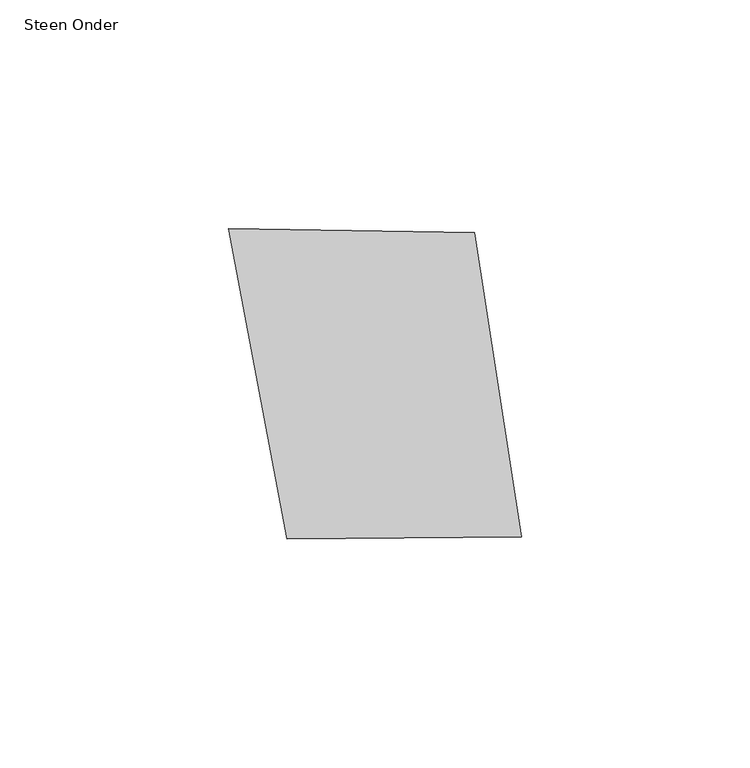
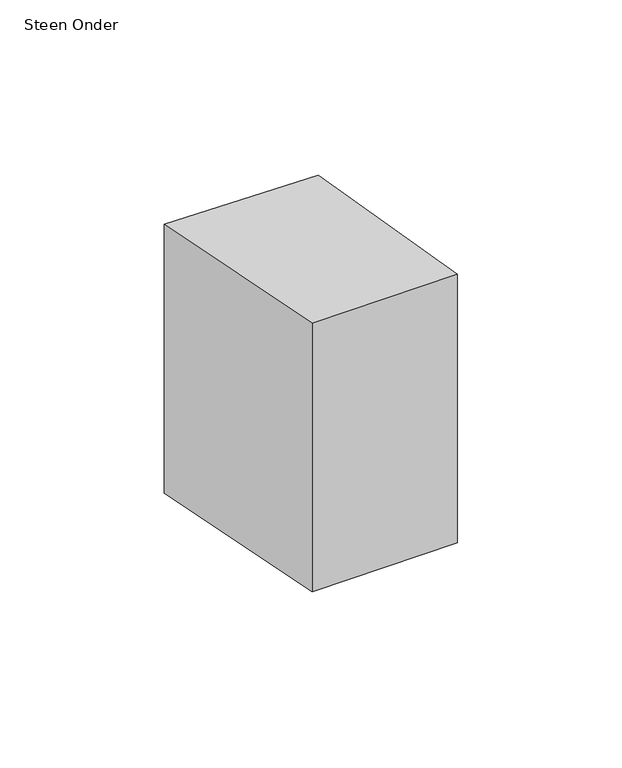
"""IFC4 building model written with IfcOpenShell, lengths in millimetres: proxy geometry, 00_GMA_steen_versie_4 : Steen Onder."""

from ifc_helpers import new_model, si_unit, origin, origin_with_axes, place, context, project, spatial, polyline, outline, extrude, source, transform, mapped, element, save


def steen_onder_d345ffee(model_context):
    return source(origin(), model_context, "Body", "SweptSolid", [
        extrude(outline(polyline([(95.7779209, 99.5138941), (106.0949539, 32.874146), (54.8034129, 32.4112295), (41.9456954, 100.3821665), (95.7779209, 99.5138941)])), origin_with_axes(), (0.0, 0.0, 1.0), 100.0),
    ])


if __name__ == "__main__":
    model = new_model("IFC4")
    model_context = context("Model", 3, world=origin())
    ifc_project = project(units=[si_unit("LENGTHUNIT", "METRE", prefix="MILLI")], contexts=[model_context])
    site = spatial("IfcSite", under=ifc_project)
    building = spatial("IfcBuilding", under=site)
    placement = place(None, origin())
    steen_onder_shape = steen_onder_d345ffee(model_context)
    element("IfcBuildingElementProxy", 1, Name="00_GMA_steen_versie_4 : Steen Onder", ObjectType="00_GMA_steen_versie_4 : Steen Onder", at=placement, inside=building, context=model_context, shape_type="MappedRepresentation", body=[
        mapped(steen_onder_shape, transform((0.0, 0.0, 0.0), x_axis=(1.0, 0.0, 0.0), y_axis=(0.0, 1.0, 0.0), z_axis=(0.0, 0.0, 1.0))),
    ])
    save(model, "model.ifc")

# Revit data of these elements
# Type "00_GMA_steen_versie_4 : Steen Onder"
#   StootVoegHalfBoven [instance default] = 5 mm
#   StootVoegHalf [instance default] = 5 mm
#   StootVoegBreedteOnder = 10 mm
#   StootVoegBreedteBoven = 10 mm
#   Steendikte = 100 mm
#   LintVoegOnderHalf = 0 mm
#   LintVoegOnder = 0 mm
#   LintVoegBovenHalf = 5 mm
#   LintVoegBoven = 10 mm
#   materiaal = none
#   MateriaalVoeg = none
#   Default Elevation = 0
